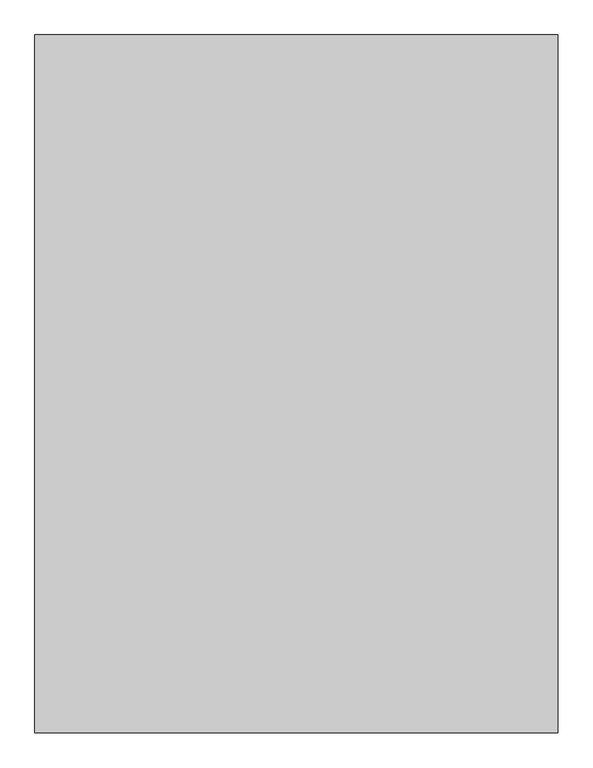
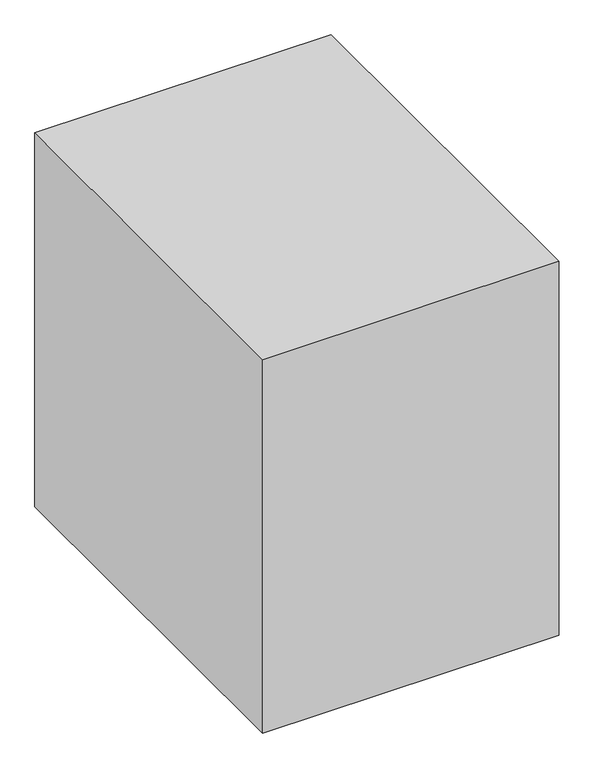
"""IFC4 building model written with IfcOpenShell, lengths in millimetres: proxy geometry, Space Planning Box_hec : Space Planning Box_hec."""

from ifc_helpers import new_model, si_unit, origin, origin_with_axes, place, context, project, spatial, polyline, outline, extrude, source, transform, mapped, element, save


def generic_models_8af91fed(model_context):
    return source(origin(), model_context, "Body", "SweptSolid", [
        extrude(outline(polyline([(2250.0, 3000.0), (2250.0, -3000.0), (-2250.0, -3000.0), (-2250.0, 3000.0), (2250.0, 3000.0)])), origin_with_axes(), (0.0, 0.0, 1.0), 6000.0),
    ])


if __name__ == "__main__":
    model = new_model("IFC4")
    model_context = context("Model", 3, world=origin())
    ifc_project = project(units=[si_unit("LENGTHUNIT", "METRE", prefix="MILLI")], contexts=[model_context])
    site = spatial("IfcSite", under=ifc_project)
    building = spatial("IfcBuilding", under=site)
    placement = place(None, origin())
    generic_models_shape = generic_models_8af91fed(model_context)
    element("IfcBuildingElementProxy", 1, Name="Space Planning Box_hec : Space Planning Box_hec", ObjectType="Space Planning Box_hec : Space Planning Box_hec", at=placement, inside=building, context=model_context, shape_type="MappedRepresentation", body=[
        mapped(generic_models_shape, transform((0.0, 0.0, 0.0), x_axis=(1.0, 0.0, 0.0), y_axis=(0.0, 1.0, 0.0), z_axis=(0.0, 0.0, 1.0))),
    ])
    save(model, "model.ifc")

# Revit data of these elements
# Type "Space Planning Box_hec : Space Planning Box_hec"
#   Type Comments = "..."
#   Room Name [instance default] = "?"
#   Interior Finish [instance default] = ""
#   Exterior Finish [instance default] = ""
#   Department [instance default] = ""
#   Assembly Code = "..."
#   Width [instance default] = 1524 mm
#   Program Area [instance default] = 0 m²
#   Length [instance default] = 1524 mm
#   Height [instance default] = 1524 mm
#   Area [instance default] = 2.32258 m²
#   Fill Color [instance default] = Cyan
#   Default Elevation = 0
# Element 1 (IfcBuildingElementProxy, "Space Planning Box_hec : Space Planning Box_hec")
#   Room Name = "Document Room"
#   Interior Finish = "IF2-1"
#   Exterior Finish = "EF1"
#   Department = "AR"
#   Width = 4500 mm
#   Program Area = 48 m²
#   Length = 6000 mm
#   Height = 6000 mm
#   Area = 27 m²
#   Fill Color = Lavender
#   Materials on its faces: "Lavender"
# Materials
#   "Cyan": class "Generic", colour RGB 0 255 255, transparency 0.2, Cost = 0
#   "Lavender": class "Generic", colour RGB 186 85 211, transparency 0.2, Cost = 0
